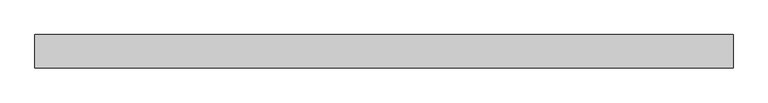
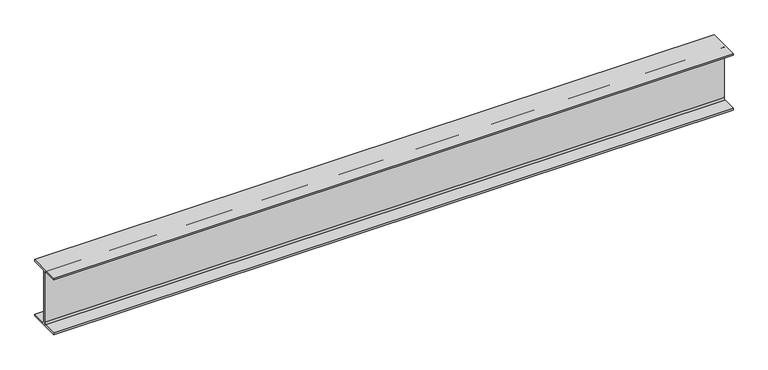
"""IFC4 building model written with IfcOpenShell, lengths in millimetres: beam geometry, Old_Steel Beam_H-KSD3502 : H_SB_ASB_H-200×200x8x12."""

from ifc_helpers import new_model, si_unit, point, frame, frame_2d, origin, place, context, project, spatial, polyline, circle_curve, trimmed, segment, composite_curve, outline, extrude, source, transform, mapped, element, save


def beam_ff0b4b27(model_context):
    return source(origin(), model_context, "Body", "SweptSolid", [
        extrude(outline(composite_curve([segment(polyline([(-82.5, -141.5), (-11.9, -141.5)]), True, "CONTINUOUS"), segment(trimmed(circle_curve(frame_2d((-11.9, -132.6)), 8.9), [point((-11.9, -141.5))], [point((-3.0, -132.6))], True, "CARTESIAN"), True, "CONTINUOUS"), segment(polyline([(-3.0, -132.6), (-3.0, 132.6)]), True, "CONTINUOUS"), segment(trimmed(circle_curve(frame_2d((-11.9, 132.6)), 8.9), [point((-3.0, 132.6))], [point((-11.9, 141.5))], True, "CARTESIAN"), True, "CONTINUOUS"), segment(polyline([(-11.9, 141.5), (-82.5, 141.5), (-82.5, 151.7), (82.5, 151.7), (82.5, 141.5), (11.9, 141.5)]), True, "CONTINUOUS"), segment(trimmed(circle_curve(frame_2d((11.9, 132.6)), 8.9), [point((11.9, 141.5))], [point((3.0, 132.6))], True, "CARTESIAN"), True, "CONTINUOUS"), segment(polyline([(3.0, 132.6), (3.0, -132.6)]), True, "CONTINUOUS"), segment(trimmed(circle_curve(frame_2d((11.9, -132.6)), 8.9), [point((3.0, -132.6))], [point((11.9, -141.5))], True, "CARTESIAN"), True, "CONTINUOUS"), segment(polyline([(11.9, -141.5), (82.5, -141.5), (82.5, -151.7), (-82.5, -151.7), (-82.5, -141.5)]), True, "CONTINUOUS")], self_intersect=False)), frame((-1737.9303669, 0.0, 0.0), z_axis=(1.0, 0.0, 0.0), x_axis=(0.0, 1.0, 0.0)), (0.0, 0.0, 1.0), 3445.4570815),
    ])


if __name__ == "__main__":
    model = new_model("IFC4")
    model_context = context("Model", 3, world=origin())
    ifc_project = project(units=[si_unit("LENGTHUNIT", "METRE", prefix="MILLI")], contexts=[model_context])
    site = spatial("IfcSite", under=ifc_project)
    building = spatial("IfcBuilding", under=site)
    placement = place(None, origin())
    beam_shape = beam_ff0b4b27(model_context)
    element("IfcBeam", 1, ObjectType="Old_Steel Beam_H-KSD3502 : H_SB_ASB_H-200×200x8x12", at=placement, inside=building, context=model_context, shape_type="MappedRepresentation", body=[
        mapped(beam_shape, transform((0.0, 0.0, 0.0), x_axis=(1.0, 0.0, 0.0), y_axis=(0.0, 1.0, 0.0), z_axis=(0.0, 0.0, 1.0))),
    ])
    save(model, "model.ifc")

# Revit data of these elements
# Type "Old_Steel Beam_H-KSD3502 : H_SB_ASB_H-200×200x8x12"
#   Width = 20.0 cm
#   Web Thickness = 0.8 cm
#   Web Fillet = 1.3 cm
#   Warping Constant = 141376.0 cm⁶
#   Torsional Moment of Inertia = 26.2485 cm⁴
#   Torsional Modulus = 1.0 cm³
#   Section Area = 63.53 cm²
#   Plastic Modulus weak axis = 244.0 cm³
#   Plastic Modulus strong axis = 525.0 cm³
#   Perimeter = 1.16 m²/m
#   Nominal Weight = 49.90 kgf/m
#   Moment of Inertia weak axis = 1600.00 cm⁴
#   Moment of Inertia strong axis = 4720.00 cm⁴
#   Height = 20.0 cm
#   Flange Thickness = 1.2 cm
#   Elastic Modulus weak axis = 160.0 cm³
#   Elastic Modulus strong axis = 472.0 cm³
#   Centroid Vertical = 10.0 cm
#   Centroid Horizontal = 10.0 cm
#   Length [instance default] = 1.5240 m
#   Structural Material [instance default] = Steel, 45-345
#   Assembly Code = ""
# Element 1 (IfcBeam, "Old_Steel Beam_H-KSD3502 : H_SB_ASB_H-200×200x8x12")
#   Structural Material = none
# Materials
#   "Steel, 45-345": class "Metal", colour RGB 189 187 185, transparency 0, Description = "Steel 345 MPa", Cost = 0
